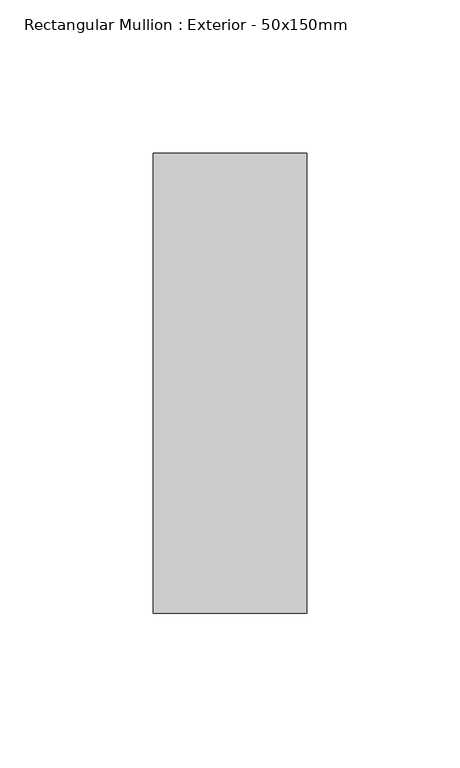
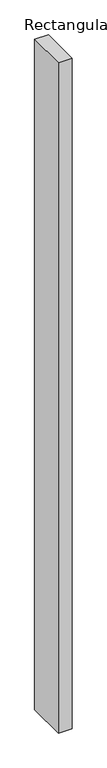
"""IFC4 building model written with IfcOpenShell, lengths in millimetres: member geometry, Rectangular Mullion : Exterior - 50x150mm."""

import ifcopenshell
import ifcopenshell.guid

model = None  # the IFC model being written
_history = None  # IfcOwnerHistory: only IFC2X3 demands one
_inside = {}  # id of a spatial element -> (the spatial element, [elements in it])
_under = {}  # id of a project, library or spatial element -> (it, [spatial elements below it])
_declared = {}  # id of a project -> (the project, [libraries it declares])
_typed = {}  # id of a type object -> (the type object, [elements of that type])
_made_of = {}  # id of a material, layer set ... -> (it, [elements and type objects made of it])


def new_model(schema):
    """Start an empty IFC model of exactly this schema.

    Asked for "IFC4X3", IfcOpenShell would pick the latest addendum, in which some entities
    have other attributes; the version numbers below select the first issue.
    IFC2X3 requires an IfcOwnerHistory on every rooted entity: one is made here for all.
    """
    global model, _history
    if schema == "IFC4X3":
        model = ifcopenshell.file(schema_version=(4, 3, 0, 0))
    else:
        model = ifcopenshell.file(schema=schema)
    _inside.clear()
    _under.clear()
    _declared.clear()
    _typed.clear()
    _made_of.clear()
    _history = None
    if model.schema == "IFC2X3":
        org = make("IfcOrganization", Name="unknown")
        user = make(
            "IfcPersonAndOrganization",
            ThePerson=make("IfcPerson", FamilyName="unknown"),
            TheOrganization=org,
        )
        app = make(
            "IfcApplication",
            ApplicationDeveloper=org,
            Version="unknown",
            ApplicationFullName="unknown",
            ApplicationIdentifier="unknown",
        )
        _history = make(
            "IfcOwnerHistory",
            OwningUser=user,
            OwningApplication=app,
            ChangeAction="ADDED",
            CreationDate=0,
        )
    return model


def make(cls, **values):
    """One entity of the class cls with the attributes given. An attribute that is None is left unset."""
    return model.create_entity(
        cls, **{name: value for name, value in values.items() if value is not None}
    )


def rooted(cls, **values):
    """An entity with a GlobalId (a new one), such as an element, a storey or a relation."""
    return make(cls, GlobalId=ifcopenshell.guid.new(), OwnerHistory=_history, **values)


def si_unit(unit_type, name, prefix=None):
    """IfcSIUnit, for example si_unit("LENGTHUNIT", "METRE", prefix="MILLI")."""
    return make("IfcSIUnit", UnitType=unit_type, Prefix=prefix, Name=name)


def assignment(units):
    """IfcUnitAssignment: the units of a project."""
    return None if units is None else make("IfcUnitAssignment", Units=units)


def point(xyz):
    """IfcCartesianPoint."""
    return None if xyz is None else make("IfcCartesianPoint", Coordinates=xyz)


def direction(xyz):
    """IfcDirection."""
    return None if xyz is None else make("IfcDirection", DirectionRatios=xyz)


def frame(location, z_axis=None, x_axis=None):
    """IfcAxis2Placement3D, a coordinate frame: its origin and axes. An axis left out is left unset."""
    return make(
        "IfcAxis2Placement3D",
        Location=point(location),
        Axis=direction(z_axis),
        RefDirection=direction(x_axis),
    )


def origin():
    """The frame at (0, 0, 0) with its axes left unset."""
    return frame((0.0, 0.0, 0.0))


def place(relative_to, where):
    """IfcLocalPlacement: puts the frame where relative to a parent placement (None: the world)."""
    return make(
        "IfcLocalPlacement", PlacementRelTo=relative_to, RelativePlacement=where
    )


def context(
    kind, dimensions, precision=None, world=None, true_north=None, identifier=None
):
    """IfcGeometricRepresentationContext, for example the 3D "Model" context."""
    return make(
        "IfcGeometricRepresentationContext",
        ContextIdentifier=identifier,
        ContextType=kind,
        CoordinateSpaceDimension=dimensions,
        Precision=precision,
        WorldCoordinateSystem=world,
        TrueNorth=true_north,
    )


def project(units=None, contexts=None):
    """IfcProject with its units and contexts."""
    return rooted(
        "IfcProject",
        Name="project",
        RepresentationContexts=contexts,
        UnitsInContext=assignment(units),
    )


def spatial(cls, under=None, at=None, **own):
    """A site, building, storey or space (cls), placed at a placement, below another one or the project."""
    s = rooted(cls, ObjectPlacement=at, **own)
    if under is not None:
        _under.setdefault(under.id(), (under, []))[1].append(s)
    return s


def polyline(points):
    """IfcPolyline through the points."""
    return make("IfcPolyline", Points=[point(p) for p in points])


def outline(outer, holes=None, kind="AREA"):
    """IfcArbitraryClosedProfileDef: a profile drawn as a closed curve; with holes, ...WithVoids."""
    if holes is None:
        return make("IfcArbitraryClosedProfileDef", ProfileType=kind, OuterCurve=outer)
    return make(
        "IfcArbitraryProfileDefWithVoids",
        ProfileType=kind,
        OuterCurve=outer,
        InnerCurves=holes,
    )


def extrude(swept, where, along, depth):
    """IfcExtrudedAreaSolid: the profile swept, set in the frame where, extruded along a direction by depth."""
    return make(
        "IfcExtrudedAreaSolid",
        SweptArea=swept,
        Position=where,
        ExtrudedDirection=direction(along),
        Depth=depth,
    )


def shape(context_of_items, identifier, shape_type, items):
    """IfcShapeRepresentation: the items that make up one representation, for example the "Body"."""
    return make(
        "IfcShapeRepresentation",
        ContextOfItems=context_of_items,
        RepresentationIdentifier=identifier,
        RepresentationType=shape_type,
        Items=items,
    )


def source(mapping_origin, context_of_items, identifier, shape_type, items):
    """IfcRepresentationMap: a shape defined once, which mapped items show again and again."""
    return make(
        "IfcRepresentationMap",
        MappingOrigin=mapping_origin,
        MappedRepresentation=shape(context_of_items, identifier, shape_type, items),
    )


def transform(
    local_origin,
    x_axis=None,
    y_axis=None,
    z_axis=None,
    scale=None,
    scale2=None,
    scale3=None,
    uniform=True,
):
    """IfcCartesianTransformationOperator3D, or its non-uniform kind. x_axis, y_axis, z_axis: its Axis1, 2, 3."""
    if uniform:
        return make(
            "IfcCartesianTransformationOperator3D",
            Axis1=direction(x_axis),
            Axis2=direction(y_axis),
            LocalOrigin=point(local_origin),
            Scale=scale,
            Axis3=direction(z_axis),
        )
    return make(
        "IfcCartesianTransformationOperator3DnonUniform",
        Axis1=direction(x_axis),
        Axis2=direction(y_axis),
        LocalOrigin=point(local_origin),
        Scale=scale,
        Axis3=direction(z_axis),
        Scale2=scale2,
        Scale3=scale3,
    )


def mapped(mapping_source, mapping_target):
    """IfcMappedItem: shows the shape of a source again, moved by a transform."""
    return make(
        "IfcMappedItem", MappingSource=mapping_source, MappingTarget=mapping_target
    )


def made_of(thing, what):
    """Note that an element or type object is made of a material, layer set ...; save() writes the relation."""
    if what is not None:
        _made_of.setdefault(what.id(), (what, []))[1].append(thing)
    return thing


def element(
    cls,
    number,
    at=None,
    inside=None,
    cuts=None,
    type_object=None,
    material=None,
    context=None,
    identifier="Body",
    shape_type=None,
    held_by="IfcProductDefinitionShape",
    body=None,
    shapes=None,
    **own,
):
    """One element of the class cls, such as IfcWall. Its Tag is "e" and its number.

    at: its placement. inside: the storey or other place that contains it. cuts: it is an
    opening in that element (IfcRelVoidsElement). A single representation is given by context,
    identifier, shape_type and body (its items); several are given by shapes. held_by: the class
    of the entity that holds the representations. save() writes the other relations.
    """
    e = rooted(cls, Tag="e%d" % number, ObjectPlacement=at, **own)
    if body is not None:
        shapes = [shape(context, identifier, shape_type, body)]
    if shapes is not None:
        e.Representation = make(held_by, Representations=shapes)
    if inside is not None:
        _inside.setdefault(inside.id(), (inside, []))[1].append(e)
    if cuts is not None:
        rooted(
            "IfcRelVoidsElement", RelatingBuildingElement=cuts, RelatedOpeningElement=e
        )
    if type_object is not None:
        _typed.setdefault(type_object.id(), (type_object, []))[1].append(e)
    return made_of(e, material)


def aggregate(whole, parts):
    """IfcRelAggregates: a whole, such as a stair, and the parts it consists of."""
    return rooted("IfcRelAggregates", RelatingObject=whole, RelatedObjects=parts)


def save(model, path):
    """Write the relations noted so far, then the file.

    IfcRelAggregates (storeys below a building ...), IfcRelContainedInSpatialStructure (elements
    in a storey), IfcRelDefinesByType, IfcRelAssociatesMaterial and IfcRelDeclares: one each for
    every whole, place, type object, material and project.
    """
    for whole, parts in _under.values():
        aggregate(whole, parts)
    for where, things in _inside.values():
        rooted(
            "IfcRelContainedInSpatialStructure",
            RelatedElements=things,
            RelatingStructure=where,
        )
    for kind, things in _typed.values():
        rooted("IfcRelDefinesByType", RelatedObjects=things, RelatingType=kind)
    for what, things in _made_of.values():
        rooted("IfcRelAssociatesMaterial", RelatedObjects=things, RelatingMaterial=what)
    for by, libraries in _declared.values():
        rooted("IfcRelDeclares", RelatingContext=by, RelatedDefinitions=libraries)
    model.write(path)


def rectangular_mullion_exterior_50x150mm_be5f20bc(model_context):
    return source(origin(), model_context, "Body", "SweptSolid", [
        extrude(outline(polyline([(25.0, 0.0), (25.0, -150.0), (-25.0, -150.0), (-25.0, 0.0), (25.0, 0.0)])), frame((0.0, 0.0, -2600.0), z_axis=(0.0, 0.0, 1.0), x_axis=(1.0, 0.0, 0.0)), (0.0, 0.0, 1.0), 2600.0),
    ])


if __name__ == "__main__":
    model = new_model("IFC4")
    model_context = context("Model", 3, world=origin())
    ifc_project = project(units=[si_unit("LENGTHUNIT", "METRE", prefix="MILLI")], contexts=[model_context])
    site = spatial("IfcSite", under=ifc_project)
    building = spatial("IfcBuilding", under=site)
    placement = place(None, origin())
    rectangular_mullion_exterior_50x150mm_shape = rectangular_mullion_exterior_50x150mm_be5f20bc(model_context)
    element("IfcMember", 1, ObjectType="Rectangular Mullion : Exterior - 50x150mm", at=placement, inside=building, context=model_context, shape_type="MappedRepresentation", body=[
        mapped(rectangular_mullion_exterior_50x150mm_shape, transform((0.0, 0.0, 0.0), x_axis=(1.0, 0.0, 0.0), y_axis=(0.0, 1.0, 0.0), z_axis=(0.0, 0.0, 1.0))),
    ])
    save(model, "model.ifc")

# Revit data of these elements
# Project information
#   Template Version = "DanEDU Building template ver. 2018.0420.0"
#   Client Name = "Test Project"
#   Project Address = "Enter address here"
#   Project Name = "3 Stories"
#   Project Number = "Number"
#   Current Version = "0.0.0"
#   SR Document GUID = "3eb9317e-835d-4f79-8926-4d15b96bc824"
# Type "Rectangular Mullion : Exterior - 50x150mm"
#   built-in parameter 1007351 = -0.246063 (stored number, unit not read)
#   built-in parameter 1007304 = 0.492126 (stored number, unit not read)
#   built-in parameter 1007301 = 0.082021 (stored number, unit not read)
#   built-in parameter 1007300 = 0.082021 (stored number, unit not read)
# Element 1 (IfcMember, "Rectangular Mullion : Exterior - 50x150mm")
#   Materials on its faces: "Default Frame/Mullion (Interior/Exterior)"
# Materials
#   "Default Frame/Mullion (Interior/Exterior)": class "Generic", colour RGB 205 205 205, transparency 0, Description = "Udefineret karm/ramme materiale", Cost = 0
